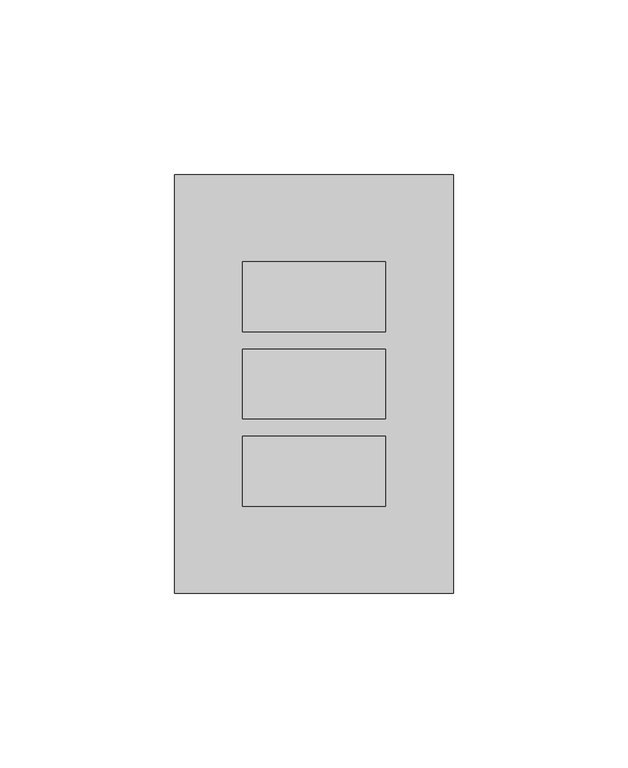
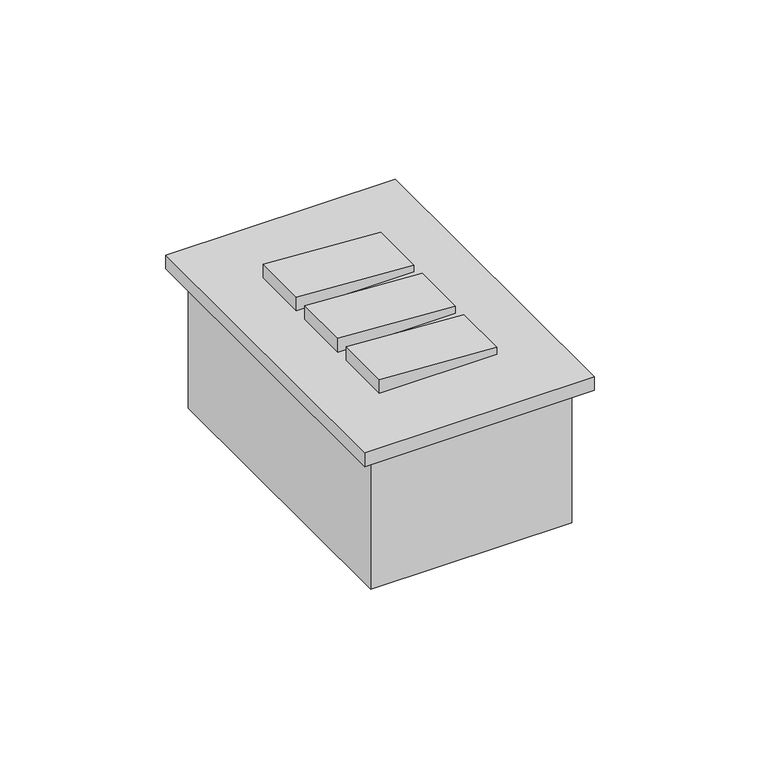
"""IFC4 building model written with IfcOpenShell, lengths in millimetres: proxy geometry, CAIXA VERTICE V7 : Interruptor 3s."""

from ifc_helpers import new_model, si_unit, frame, origin, origin_with_axes, place, context, project, spatial, polyline, outline, extrude, faceted_brep, source, transform, mapped, element, save


def electrical_fixtures_ba972305(model_context):
    return source(origin(), model_context, "Body", "SolidModel", [
        extrude(outline(polyline([(5.0, 20.5), (7.5, 20.5), (10.0, -20.5), (5.0, -20.5), (5.0, 20.5)])), frame((0.0, 1065.0, 0.0), z_axis=(0.0, 1.0, 0.0), x_axis=(0.0, 0.0, 1.0)), (0.0, 0.0, 1.0), 20.0),
        extrude(outline(polyline([(5.0, 20.5), (7.5, 20.5), (10.0, -20.5), (5.0, -20.5), (5.0, 20.5)])), frame((0.0, 1090.0, 0.0), z_axis=(0.0, 1.0, 0.0), x_axis=(0.0, 0.0, 1.0)), (0.0, 0.0, 1.0), 20.0),
        extrude(outline(polyline([(5.0, 20.5), (7.5, 20.5), (10.0, -20.5), (5.0, -20.5), (5.0, 20.5)])), frame((0.0, 1115.0, 0.0), z_axis=(0.0, 1.0, 0.0), x_axis=(0.0, 0.0, 1.0)), (0.0, 0.0, 1.0), 20.0),
        faceted_brep([(33.0, 1047.0, -48.0), (33.0, 1153.0, -48.0), (-33.0, 1153.0, -48.0), (-33.0, 1047.0, -48.0), (35.0, 1155.0, -50.0), (35.0, 1045.0, -50.0), (-35.0, 1045.0, -50.0), (-35.0, 1155.0, -50.0), (-35.0, 1155.0, 0.0), (35.0, 1155.0, 0.0), (-35.0, 1045.0, 0.0), (35.0, 1045.0, 0.0), (33.0, 1153.0, 0.0), (33.0, 1047.0, 0.0), (-33.0, 1047.0, 0.0), (-33.0, 1153.0, 0.0)], [[[0, 1, 2, 3]], [[4, 5, 6, 7]], [[4, 7, 8, 9]], [[8, 7, 6, 10]], [[10, 6, 5, 11]], [[11, 5, 4, 9]], [[9, 8, 10, 11], [12, 13, 14, 15]], [[13, 12, 1, 0]], [[14, 13, 0, 3]], [[15, 14, 3, 2]], [[12, 15, 2, 1]]]),
        extrude(outline(polyline([(40.0, 1160.0), (40.0, 1040.0), (-40.0, 1040.0), (-40.0, 1160.0), (40.0, 1160.0)])), origin_with_axes(), (0.0, 0.0, 1.0), 5.0),
    ])


if __name__ == "__main__":
    model = new_model("IFC4")
    model_context = context("Model", 3, world=origin())
    ifc_project = project(units=[si_unit("LENGTHUNIT", "METRE", prefix="MILLI")], contexts=[model_context])
    site = spatial("IfcSite", under=ifc_project)
    building = spatial("IfcBuilding", under=site)
    placement = place(None, origin())
    electrical_fixtures_shape = electrical_fixtures_ba972305(model_context)
    element("IfcBuildingElementProxy", 1, Name="CAIXA VERTICE V7 : Interruptor 3s", ObjectType="CAIXA VERTICE V7 : Interruptor 3s", at=placement, inside=building, context=model_context, shape_type="MappedRepresentation", body=[
        mapped(electrical_fixtures_shape, transform((0.0, 0.0, 0.0), x_axis=(1.0, 0.0, 0.0), y_axis=(0.0, 1.0, 0.0), z_axis=(0.0, 0.0, 1.0))),
    ])
    save(model, "model.ifc")

# Revit data of these elements
# Type "CAIXA VERTICE V7 : Interruptor 3s"
#   URL = "www.facebook.com/verticetreinamentos"
#   SEÇÃO [instance default] = ""
#   Rotação [instance default] = 0.00°
#   LARGURA DA TAMPA = 0.08 m
#   BORDA = 0.01 m
#   ALTURA DE INSTALAÇÃO [instance default] = 1.10 m
#   Distância Anotação [instance default] = 0.0015 m
#   ALTURA DA TAMPA = 0.12 m
#   Vertical [instance default] = yes
#   VER SEÇÃO [instance default] = yes
#   SHADE ESQ [instance default] = no
#   SHADE DIR [instance default] = yes
#   HORIZONTAL [instance default] = no
#   ANDAR COM A LEGENDA [instance default] = 0
#   Material Tampa [instance default] = Plástico, branco opaco
#   Caixa = element 1798511
#   Anotação = element 1798523
#   Default Elevation = 0
# Element 1 (IfcBuildingElementProxy, "CAIXA VERTICE V7 : Interruptor 3s")
#   SEÇÃO = "3"
#   Distância Anotação = 0.0055 m
#   ANDAR COM A LEGENDA = 2
#   Materials on its faces: "Plástico, branco opaco"
# Materials
#   "Plástico, branco opaco": class "Plástico", colour RGB 120 120 120, transparency 0, Description = "Plastic, generic, opaque white", Cost = 0
